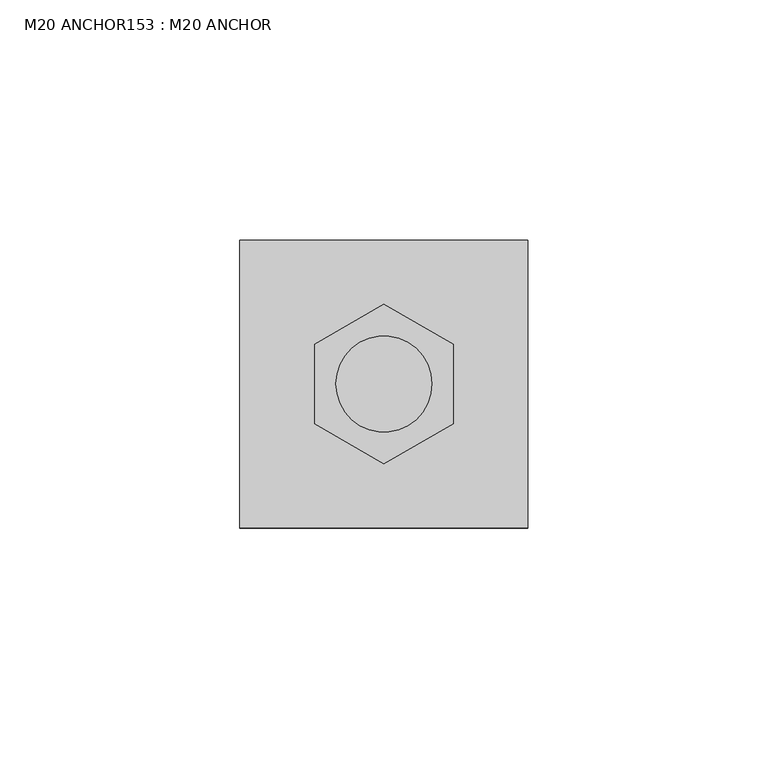
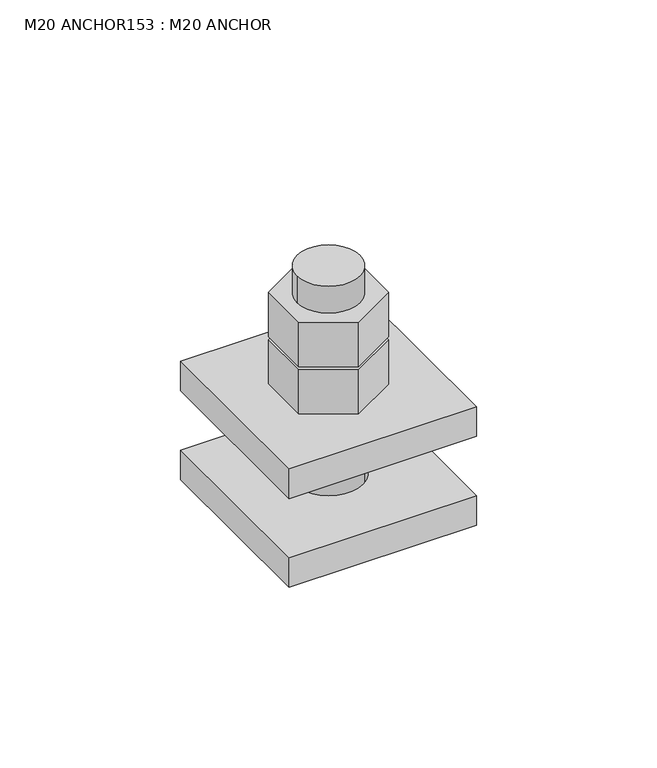
"""IFC4 building model written with IfcOpenShell, lengths in millimetres: fastener geometry, M20 ANCHOR153 : M20 ANCHOR."""

from ifc_helpers import new_model, si_unit, point, frame, frame_2d, origin, place, context, project, spatial, polyline, circle_curve, trimmed, segment, composite_curve, outline, extrude, source, transform, mapped, element, save


def m20_anchor153_m20_anchor_955b5c47(model_context):
    return source(origin(), model_context, "Body", "SweptSolid", [
        extrude(outline(polyline([(5991.9144032, 25545.0952779), (5991.9144032, 25528.4582151), (5977.5062842, 25520.1396837), (5963.0981652, 25528.4582151), (5963.0981652, 25545.0952779), (5977.5062842, 25553.4138093), (5991.9144032, 25545.0952779)]), holes=[composite_curve([segment(trimmed(circle_curve(frame_2d((5977.5062842, 25536.7767465)), 10.0), [point((5967.5062842, 25536.7767465))], [point((5987.5062842, 25536.7767465))], True, "CARTESIAN"), True, "CONTINUOUS"), segment(trimmed(circle_curve(frame_2d((5977.5062842, 25536.7767465)), 10.0), [point((5987.5062842, 25536.7767465))], [point((5967.5062842, 25536.7767465))], True, "CARTESIAN"), True, "CONTINUOUS")], self_intersect=False)]), frame((0.0, 0.0, 246.0), z_axis=(0.0, 0.0, 1.0), x_axis=(1.0, 0.0, 0.0)), (0.0, 0.0, 1.0), 15.0),
        extrude(outline(polyline([(5991.9144032, 25545.0952779), (5991.9144032, 25528.4582151), (5977.5062842, 25520.1396837), (5963.0981652, 25528.4582151), (5963.0981652, 25545.0952779), (5977.5062842, 25553.4138093), (5991.9144032, 25545.0952779)]), holes=[composite_curve([segment(trimmed(circle_curve(frame_2d((5977.5062842, 25536.7767465)), 10.0), [point((5967.5062842, 25536.7767465))], [point((5987.5062842, 25536.7767465))], True, "CARTESIAN"), True, "CONTINUOUS"), segment(trimmed(circle_curve(frame_2d((5977.5062842, 25536.7767465)), 10.0), [point((5987.5062842, 25536.7767465))], [point((5967.5062842, 25536.7767465))], True, "CARTESIAN"), True, "CONTINUOUS")], self_intersect=False)]), frame((0.0, 0.0, 230.0), z_axis=(0.0, 0.0, 1.0), x_axis=(1.0, 0.0, 0.0)), (0.0, 0.0, 1.0), 15.0),
        extrude(outline(composite_curve([segment(trimmed(circle_curve(frame_2d((5977.5062842, 25536.7767465)), 10.0), [point((5967.5062842, 25536.7767465))], [point((5987.5062842, 25536.7767465))], False, "CARTESIAN"), True, "CONTINUOUS"), segment(trimmed(circle_curve(frame_2d((5977.5062842, 25536.7767465)), 10.0), [point((5987.5062842, 25536.7767465))], [point((5967.5062842, 25536.7767465))], False, "CARTESIAN"), True, "CONTINUOUS")], self_intersect=False)), frame((0.0, 0.0, 190.0), z_axis=(0.0, 0.0, 1.0), x_axis=(1.0, 0.0, 0.0)), (0.0, 0.0, 1.0), 80.0),
        extrude(outline(polyline([(6007.5062842, 25566.7767465), (6007.5062842, 25506.7767465), (5947.5062842, 25506.7767465), (5947.5062842, 25566.7767465), (6007.5062842, 25566.7767465)]), holes=[composite_curve([segment(trimmed(circle_curve(frame_2d((5977.5062842, 25536.7767465)), 11.0), [point((5966.5062842, 25536.7767465))], [point((5988.5062842, 25536.7767465))], True, "CARTESIAN"), True, "CONTINUOUS"), segment(trimmed(circle_curve(frame_2d((5977.5062842, 25536.7767465)), 11.0), [point((5988.5062842, 25536.7767465))], [point((5966.5062842, 25536.7767465))], True, "CARTESIAN"), True, "CONTINUOUS")], self_intersect=False)]), frame((0.0, 0.0, 190.0), z_axis=(0.0, 0.0, 1.0), x_axis=(1.0, 0.0, 0.0)), (0.0, 0.0, 1.0), 10.0),
        extrude(outline(polyline([(6007.5062842, 25566.7767465), (6007.5062842, 25506.7767465), (5947.5062842, 25506.7767465), (5947.5062842, 25566.7767465), (6007.5062842, 25566.7767465)]), holes=[composite_curve([segment(trimmed(circle_curve(frame_2d((5977.5062842, 25536.7767465)), 11.0), [point((5966.5062842, 25536.7767465))], [point((5988.5062842, 25536.7767465))], True, "CARTESIAN"), True, "CONTINUOUS"), segment(trimmed(circle_curve(frame_2d((5977.5062842, 25536.7767465)), 11.0), [point((5988.5062842, 25536.7767465))], [point((5966.5062842, 25536.7767465))], True, "CARTESIAN"), True, "CONTINUOUS")], self_intersect=False)]), frame((0.0, 0.0, 220.0), z_axis=(0.0, 0.0, 1.0), x_axis=(1.0, 0.0, 0.0)), (0.0, 0.0, 1.0), 10.0),
    ])


if __name__ == "__main__":
    model = new_model("IFC4")
    model_context = context("Model", 3, world=origin())
    ifc_project = project(units=[si_unit("LENGTHUNIT", "METRE", prefix="MILLI")], contexts=[model_context])
    site = spatial("IfcSite", under=ifc_project)
    building = spatial("IfcBuilding", under=site)
    placement = place(None, origin())
    m20_anchor153_m20_anchor_shape = m20_anchor153_m20_anchor_955b5c47(model_context)
    element("IfcFastener", 1, ObjectType="M20 ANCHOR153 : M20 ANCHOR", at=placement, inside=building, context=model_context, shape_type="MappedRepresentation", body=[
        mapped(m20_anchor153_m20_anchor_shape, transform((0.0, 0.0, 0.0), x_axis=(1.0, 0.0, 0.0), y_axis=(0.0, 1.0, 0.0), z_axis=(0.0, 0.0, 1.0))),
    ])
    save(model, "model.ifc")
